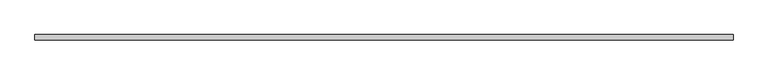
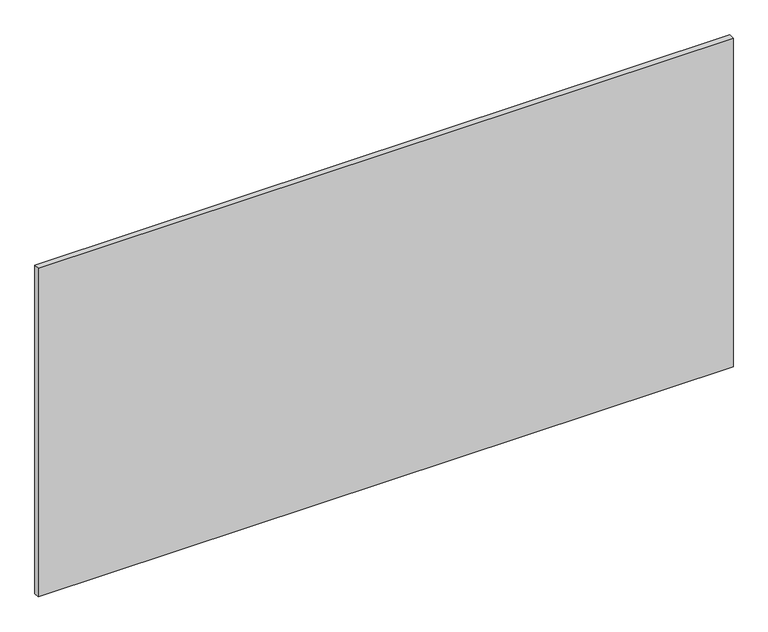
"""IFC4 building model written with IfcOpenShell, lengths in millimetres: proxy geometry, Inner panel:Inner panel:1:Inner panel:1 : Inner panel:Inner panel:300324:300043:Inner panel:1:Inner panel:1 : Inner panel:Inner panel:300324:300043 : Inner panel:Inner panel:1:Inner panel:1 : Inner panel:Inner panel:300324:300043:18 : Inner panel:Inner panel:1:Inner panel:1 : Inner panel:Inner panel:300324:300043:Inner panel:1:Inner panel:1 : Inner panel:Inner panel:300324:300043 : Inner panel:Inner panel:1:Inner panel:1 : Inner panel:Inner panel:300324:300043:300031."""

from ifc_helpers import new_model, si_unit, frame, origin, place, context, project, spatial, polyline, outline, extrude, source, transform, mapped, element, save


def generic_models_95cf7f47(model_context):
    return source(origin(), model_context, "Body", "SweptSolid", [
        extrude(outline(polyline([(591293.3367236, -568186.6413841), (593731.7367236, -568186.6413841), (593731.7367236, -568205.6913841), (591293.3367236, -568205.6913841), (591293.3367236, -568186.6413841)])), frame((0.0, 0.0, 2495.55), z_axis=(0.0, 0.0, 1.0), x_axis=(1.0, 0.0, 0.0)), (0.0, 0.0, 1.0), 1219.2),
    ])


if __name__ == "__main__":
    model = new_model("IFC4")
    model_context = context("Model", 3, world=origin())
    ifc_project = project(units=[si_unit("LENGTHUNIT", "METRE", prefix="MILLI")], contexts=[model_context])
    site = spatial("IfcSite", under=ifc_project)
    building = spatial("IfcBuilding", under=site)
    placement = place(None, origin())
    generic_models_shape = generic_models_95cf7f47(model_context)
    element("IfcBuildingElementProxy", 1, Name="Inner panel:Inner panel:1:Inner panel:1 : Inner panel:Inner panel:300324:300043:Inner panel:1:Inner panel:1 : Inner panel:Inner panel:300324:300043 : Inner panel:Inner panel:1:Inner panel:1 : Inner panel:Inner panel:300324:300043:18 : Inner panel:Inner panel:1:Inner panel:1 : Inner panel:Inner panel:300324:300043:Inner panel:1:Inner panel:1 : Inner panel:Inner panel:300324:300043 : Inner panel:Inner panel:1:Inner panel:1 : Inner panel:Inner panel:300324:300043:300031", ObjectType="Inner panel:Inner panel:1:Inner panel:1 : Inner panel:Inner panel:300324:300043:Inner panel:1:Inner panel:1 : Inner panel:Inner panel:300324:300043 : Inner panel:Inner panel:1:Inner panel:1 : Inner panel:Inner panel:300324:300043:18 : Inner panel:Inner panel:1:Inner panel:1 : Inner panel:Inner panel:300324:300043:Inner panel:1:Inner panel:1 : Inner panel:Inner panel:300324:300043 : Inner panel:Inner panel:1:Inner panel:1 : Inner panel:Inner panel:300324:300043:300031", at=placement, inside=building, context=model_context, shape_type="MappedRepresentation", body=[
        mapped(generic_models_shape, transform((0.0, 0.0, 0.0), x_axis=(1.0, 0.0, 0.0), y_axis=(0.0, 1.0, 0.0), z_axis=(0.0, 0.0, 1.0))),
    ])
    save(model, "model.ifc")

# Revit data of these elements
# Type "Inner panel:Inner panel:1:Inner panel:1 : Inner panel:Inner panel:300324:300043:Inner panel:1:Inner panel:1 : Inner panel:Inner panel:300324:300043 : Inner panel:Inner panel:1:Inner panel:1 : Inner panel:Inner panel:300324:300043:18 : Inner panel:Inner panel:1:Inner panel:1 : Inner panel:Inner panel:300324:300043:Inner panel:1:Inner panel:1 : Inner panel:Inner panel:300324:300043 : Inner panel:Inner panel:1:Inner panel:1 : Inner panel:Inner panel:300324:300043:300031"
#   NameOverride = "Inner panel:Inner panel:1:Inner panel:1 : Inner panel:Inner panel:300324:300043:Inner panel:1:Inner panel:1 : Inner panel:Inner panel:300324:300043 : Inner panel:Inner panel:1:Inner panel:1 : Inner panel:Inner panel:300324:300043:300031"
#   ObjectTypeOverride = "Inner panel:1:Inner panel:1 : Inner panel:Inner panel:300324:300043 : Inner panel:Inner panel:1:Inner panel:1 : Inner panel:Inner panel:300324:300043"
#   Reference = "Inner panel"
#   Tag = "300031"
# Element 1 (IfcBuildingElementProxy, "Inner panel:Inner panel:1:Inner panel:1 : Inner panel:Inner panel:300324:300043:Inner panel:1:Inner panel:1 : Inner panel:Inner panel:300324:300043 : Inner panel:Inner panel:1:Inner panel:1 : Inner panel:Inner panel:300324:300043:18 : Inner panel:Inner panel:1:Inner panel:1 : Inner panel:Inner panel:300324:300043:Inner panel:1:Inner panel:1 : Inner panel:Inner panel:300324:300043 : Inner panel:Inner panel:1:Inner panel:1 : Inner panel:Inner panel:300324:300043:300031")
#   Materials on its faces: "¾” (CLASS A) FIRE RETARDANT PLYWOOD ...OR… IF 1/4\" GYP. BD UNDER PLYWOOD, FLAME SPREAD TO BE CLASS C -  (FINISH: GRADE B - PREFINISHED STAINED/SEALED) - 1/4\" GAP BTWN PANELS (FASTENERS T.B.D.)"
# Materials
#   "¾” (CLASS A) FIRE RETARDANT PLYWOOD ...OR… IF 1/4\" GYP. BD UNDER PLYWOOD, FLAME SPREAD TO BE CLASS C -  (FINISH: GRADE B - PREFINISHED STAINED/SEALED) - 1/4\" GAP BTWN PANELS (FASTENERS T.B.D.)": class "Wood", colour RGB 149 120 74, transparency 0, Description = "Plywood, sheathing grade", Cost = 0
